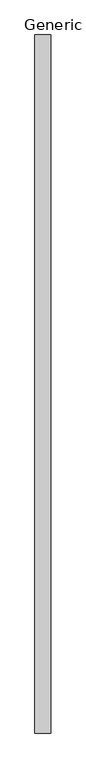
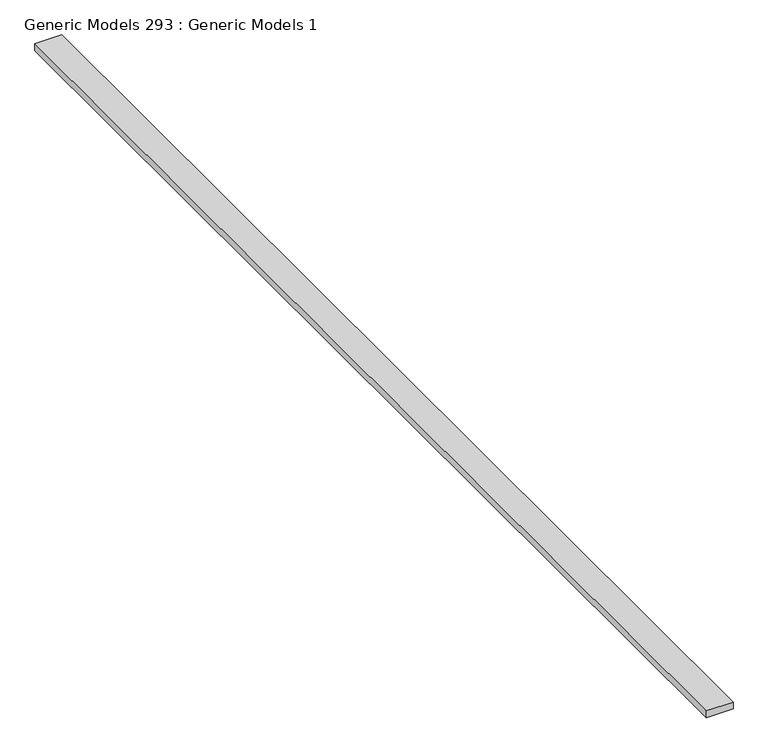
"""IFC4 building model written with IfcOpenShell, lengths in millimetres: proxy geometry, Generic Models 293 : Generic Models 1."""

import ifcopenshell
import ifcopenshell.guid

model = None  # the IFC model being written
_history = None  # IfcOwnerHistory: only IFC2X3 demands one
_inside = {}  # id of a spatial element -> (the spatial element, [elements in it])
_under = {}  # id of a project, library or spatial element -> (it, [spatial elements below it])
_declared = {}  # id of a project -> (the project, [libraries it declares])
_typed = {}  # id of a type object -> (the type object, [elements of that type])
_made_of = {}  # id of a material, layer set ... -> (it, [elements and type objects made of it])


def new_model(schema):
    """Start an empty IFC model of exactly this schema.

    Asked for "IFC4X3", IfcOpenShell would pick the latest addendum, in which some entities
    have other attributes; the version numbers below select the first issue.
    IFC2X3 requires an IfcOwnerHistory on every rooted entity: one is made here for all.
    """
    global model, _history
    if schema == "IFC4X3":
        model = ifcopenshell.file(schema_version=(4, 3, 0, 0))
    else:
        model = ifcopenshell.file(schema=schema)
    _inside.clear()
    _under.clear()
    _declared.clear()
    _typed.clear()
    _made_of.clear()
    _history = None
    if model.schema == "IFC2X3":
        org = make("IfcOrganization", Name="unknown")
        user = make(
            "IfcPersonAndOrganization",
            ThePerson=make("IfcPerson", FamilyName="unknown"),
            TheOrganization=org,
        )
        app = make(
            "IfcApplication",
            ApplicationDeveloper=org,
            Version="unknown",
            ApplicationFullName="unknown",
            ApplicationIdentifier="unknown",
        )
        _history = make(
            "IfcOwnerHistory",
            OwningUser=user,
            OwningApplication=app,
            ChangeAction="ADDED",
            CreationDate=0,
        )
    return model


def make(cls, **values):
    """One entity of the class cls with the attributes given. An attribute that is None is left unset."""
    return model.create_entity(
        cls, **{name: value for name, value in values.items() if value is not None}
    )


def rooted(cls, **values):
    """An entity with a GlobalId (a new one), such as an element, a storey or a relation."""
    return make(cls, GlobalId=ifcopenshell.guid.new(), OwnerHistory=_history, **values)


def si_unit(unit_type, name, prefix=None):
    """IfcSIUnit, for example si_unit("LENGTHUNIT", "METRE", prefix="MILLI")."""
    return make("IfcSIUnit", UnitType=unit_type, Prefix=prefix, Name=name)


def assignment(units):
    """IfcUnitAssignment: the units of a project."""
    return None if units is None else make("IfcUnitAssignment", Units=units)


def point(xyz):
    """IfcCartesianPoint."""
    return None if xyz is None else make("IfcCartesianPoint", Coordinates=xyz)


def direction(xyz):
    """IfcDirection."""
    return None if xyz is None else make("IfcDirection", DirectionRatios=xyz)


def frame(location, z_axis=None, x_axis=None):
    """IfcAxis2Placement3D, a coordinate frame: its origin and axes. An axis left out is left unset."""
    return make(
        "IfcAxis2Placement3D",
        Location=point(location),
        Axis=direction(z_axis),
        RefDirection=direction(x_axis),
    )


def origin():
    """The frame at (0, 0, 0) with its axes left unset."""
    return frame((0.0, 0.0, 0.0))


def place(relative_to, where):
    """IfcLocalPlacement: puts the frame where relative to a parent placement (None: the world)."""
    return make(
        "IfcLocalPlacement", PlacementRelTo=relative_to, RelativePlacement=where
    )


def context(
    kind, dimensions, precision=None, world=None, true_north=None, identifier=None
):
    """IfcGeometricRepresentationContext, for example the 3D "Model" context."""
    return make(
        "IfcGeometricRepresentationContext",
        ContextIdentifier=identifier,
        ContextType=kind,
        CoordinateSpaceDimension=dimensions,
        Precision=precision,
        WorldCoordinateSystem=world,
        TrueNorth=true_north,
    )


def project(units=None, contexts=None):
    """IfcProject with its units and contexts."""
    return rooted(
        "IfcProject",
        Name="project",
        RepresentationContexts=contexts,
        UnitsInContext=assignment(units),
    )


def spatial(cls, under=None, at=None, **own):
    """A site, building, storey or space (cls), placed at a placement, below another one or the project."""
    s = rooted(cls, ObjectPlacement=at, **own)
    if under is not None:
        _under.setdefault(under.id(), (under, []))[1].append(s)
    return s


def polyline(points):
    """IfcPolyline through the points."""
    return make("IfcPolyline", Points=[point(p) for p in points])


def outline(outer, holes=None, kind="AREA"):
    """IfcArbitraryClosedProfileDef: a profile drawn as a closed curve; with holes, ...WithVoids."""
    if holes is None:
        return make("IfcArbitraryClosedProfileDef", ProfileType=kind, OuterCurve=outer)
    return make(
        "IfcArbitraryProfileDefWithVoids",
        ProfileType=kind,
        OuterCurve=outer,
        InnerCurves=holes,
    )


def extrude(swept, where, along, depth):
    """IfcExtrudedAreaSolid: the profile swept, set in the frame where, extruded along a direction by depth."""
    return make(
        "IfcExtrudedAreaSolid",
        SweptArea=swept,
        Position=where,
        ExtrudedDirection=direction(along),
        Depth=depth,
    )


def shape(context_of_items, identifier, shape_type, items):
    """IfcShapeRepresentation: the items that make up one representation, for example the "Body"."""
    return make(
        "IfcShapeRepresentation",
        ContextOfItems=context_of_items,
        RepresentationIdentifier=identifier,
        RepresentationType=shape_type,
        Items=items,
    )


def source(mapping_origin, context_of_items, identifier, shape_type, items):
    """IfcRepresentationMap: a shape defined once, which mapped items show again and again."""
    return make(
        "IfcRepresentationMap",
        MappingOrigin=mapping_origin,
        MappedRepresentation=shape(context_of_items, identifier, shape_type, items),
    )


def transform(
    local_origin,
    x_axis=None,
    y_axis=None,
    z_axis=None,
    scale=None,
    scale2=None,
    scale3=None,
    uniform=True,
):
    """IfcCartesianTransformationOperator3D, or its non-uniform kind. x_axis, y_axis, z_axis: its Axis1, 2, 3."""
    if uniform:
        return make(
            "IfcCartesianTransformationOperator3D",
            Axis1=direction(x_axis),
            Axis2=direction(y_axis),
            LocalOrigin=point(local_origin),
            Scale=scale,
            Axis3=direction(z_axis),
        )
    return make(
        "IfcCartesianTransformationOperator3DnonUniform",
        Axis1=direction(x_axis),
        Axis2=direction(y_axis),
        LocalOrigin=point(local_origin),
        Scale=scale,
        Axis3=direction(z_axis),
        Scale2=scale2,
        Scale3=scale3,
    )


def mapped(mapping_source, mapping_target):
    """IfcMappedItem: shows the shape of a source again, moved by a transform."""
    return make(
        "IfcMappedItem", MappingSource=mapping_source, MappingTarget=mapping_target
    )


def made_of(thing, what):
    """Note that an element or type object is made of a material, layer set ...; save() writes the relation."""
    if what is not None:
        _made_of.setdefault(what.id(), (what, []))[1].append(thing)
    return thing


def element(
    cls,
    number,
    at=None,
    inside=None,
    cuts=None,
    type_object=None,
    material=None,
    context=None,
    identifier="Body",
    shape_type=None,
    held_by="IfcProductDefinitionShape",
    body=None,
    shapes=None,
    **own,
):
    """One element of the class cls, such as IfcWall. Its Tag is "e" and its number.

    at: its placement. inside: the storey or other place that contains it. cuts: it is an
    opening in that element (IfcRelVoidsElement). A single representation is given by context,
    identifier, shape_type and body (its items); several are given by shapes. held_by: the class
    of the entity that holds the representations. save() writes the other relations.
    """
    e = rooted(cls, Tag="e%d" % number, ObjectPlacement=at, **own)
    if body is not None:
        shapes = [shape(context, identifier, shape_type, body)]
    if shapes is not None:
        e.Representation = make(held_by, Representations=shapes)
    if inside is not None:
        _inside.setdefault(inside.id(), (inside, []))[1].append(e)
    if cuts is not None:
        rooted(
            "IfcRelVoidsElement", RelatingBuildingElement=cuts, RelatedOpeningElement=e
        )
    if type_object is not None:
        _typed.setdefault(type_object.id(), (type_object, []))[1].append(e)
    return made_of(e, material)


def aggregate(whole, parts):
    """IfcRelAggregates: a whole, such as a stair, and the parts it consists of."""
    return rooted("IfcRelAggregates", RelatingObject=whole, RelatedObjects=parts)


def save(model, path):
    """Write the relations noted so far, then the file.

    IfcRelAggregates (storeys below a building ...), IfcRelContainedInSpatialStructure (elements
    in a storey), IfcRelDefinesByType, IfcRelAssociatesMaterial and IfcRelDeclares: one each for
    every whole, place, type object, material and project.
    """
    for whole, parts in _under.values():
        aggregate(whole, parts)
    for where, things in _inside.values():
        rooted(
            "IfcRelContainedInSpatialStructure",
            RelatedElements=things,
            RelatingStructure=where,
        )
    for kind, things in _typed.values():
        rooted("IfcRelDefinesByType", RelatedObjects=things, RelatingType=kind)
    for what, things in _made_of.values():
        rooted("IfcRelAssociatesMaterial", RelatedObjects=things, RelatingMaterial=what)
    for by, libraries in _declared.values():
        rooted("IfcRelDeclares", RelatingContext=by, RelatedDefinitions=libraries)
    model.write(path)


def generic_models_293_generic_models_1_ed934f8d(model_context):
    return source(origin(), model_context, "Body", "SweptSolid", [
        extrude(outline(polyline([(6711.7763704, 11981.8769662), (6851.4763704, 11981.8769662), (6851.4763704, 5885.8769662), (6711.7763704, 5885.8769662), (6711.7763704, 11981.8769662)])), frame((0.0, 0.0, 123424.696), z_axis=(0.0, 0.0, 1.0), x_axis=(1.0, 0.0, 0.0)), (0.0, 0.0, 1.0), 38.1),
    ])


if __name__ == "__main__":
    model = new_model("IFC4")
    model_context = context("Model", 3, world=origin())
    ifc_project = project(units=[si_unit("LENGTHUNIT", "METRE", prefix="MILLI")], contexts=[model_context])
    site = spatial("IfcSite", under=ifc_project)
    building = spatial("IfcBuilding", under=site)
    placement = place(None, origin())
    generic_models_293_generic_models_1_shape = generic_models_293_generic_models_1_ed934f8d(model_context)
    element("IfcBuildingElementProxy", 1, Name="Generic Models 293 : Generic Models 1", ObjectType="Generic Models 293 : Generic Models 1", at=placement, inside=building, context=model_context, shape_type="MappedRepresentation", body=[
        mapped(generic_models_293_generic_models_1_shape, transform((0.0, 0.0, 0.0), x_axis=(1.0, 0.0, 0.0), y_axis=(0.0, 1.0, 0.0), z_axis=(0.0, 0.0, 1.0))),
    ])
    save(model, "model.ifc")

# Revit data of these elements
# Element 1 (IfcBuildingElementProxy, "Generic Models 293 : Generic Models 1")
#   Materials on its faces: "_TREATED BLOCKING AS REQUIRED"
# Materials
#   "_TREATED BLOCKING AS REQUIRED": class "Generic", colour RGB 177 130 114, transparency 0, Cost = 0
